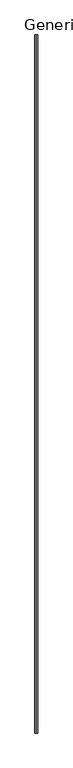
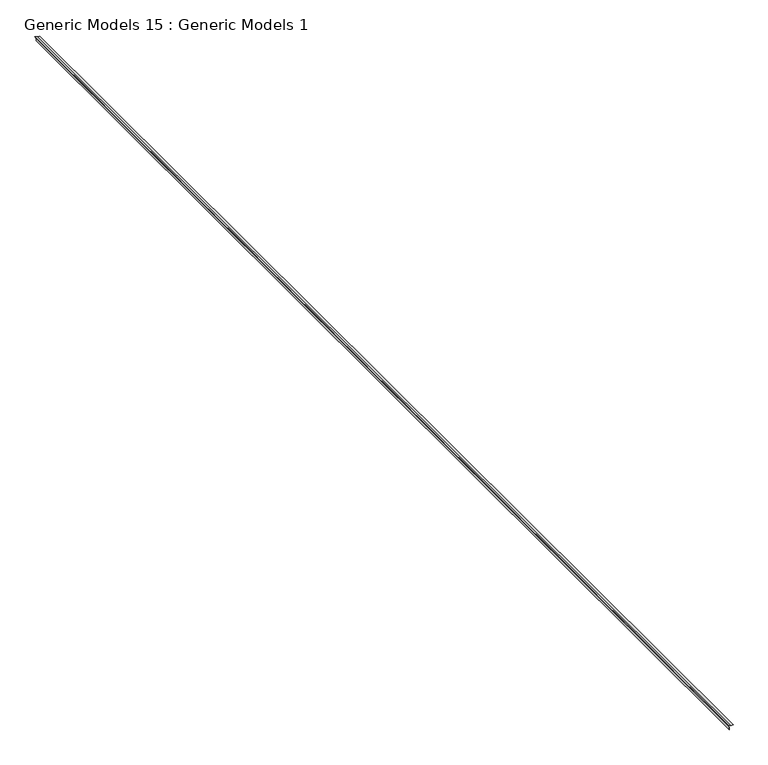
"""IFC4 building model written with IfcOpenShell, lengths in millimetres: proxy geometry, Generic Models 15 : Generic Models 1."""

from ifc_helpers import new_model, si_unit, point, frame, frame_2d, origin, place, context, project, spatial, polyline, circle_curve, trimmed, segment, composite_curve, outline, extrude, source, transform, mapped, element, save


def generic_models_15_generic_models_1_eb5eed79(model_context):
    return source(origin(), model_context, "Body", "SweptSolid", [
        extrude(outline(composite_curve([segment(trimmed(circle_curve(frame_2d((127127.2167873, 8355.8457008)), 1.4342127), [point((127128.4926156, 8356.5008558))], [point((127126.5616323, 8354.5698725))], False, "CARTESIAN"), True, "CONTINUOUS"), segment(polyline([(127126.5616323, 8354.5698725), (127088.5361176, 8374.0964881), (127050.4361176, 8374.0964881), (127050.4361176, 8375.3664881), (127088.8431414, 8375.3664881), (127127.5962396, 8355.4662484), (127107.696, 8394.2193467), (127107.696, 8432.6263704), (127108.966, 8432.6263704), (127108.966, 8394.5263704), (127128.4926156, 8356.5008558)]), True, "CONTINUOUS")], self_intersect=False)), frame((0.0, -7068.1230338, 0.0), z_axis=(0.0, 1.0, 0.0), x_axis=(0.0, 0.0, 1.0)), (0.0, 0.0, 1.0), 19050.0),
    ])


if __name__ == "__main__":
    model = new_model("IFC4")
    model_context = context("Model", 3, world=origin())
    ifc_project = project(units=[si_unit("LENGTHUNIT", "METRE", prefix="MILLI")], contexts=[model_context])
    site = spatial("IfcSite", under=ifc_project)
    building = spatial("IfcBuilding", under=site)
    placement = place(None, origin())
    generic_models_15_generic_models_1_shape = generic_models_15_generic_models_1_eb5eed79(model_context)
    element("IfcBuildingElementProxy", 1, Name="Generic Models 15 : Generic Models 1", ObjectType="Generic Models 15 : Generic Models 1", at=placement, inside=building, context=model_context, shape_type="MappedRepresentation", body=[
        mapped(generic_models_15_generic_models_1_shape, transform((0.0, 0.0, 0.0), x_axis=(1.0, 0.0, 0.0), y_axis=(0.0, 1.0, 0.0), z_axis=(0.0, 0.0, 1.0))),
    ])
    save(model, "model.ifc")

# Revit data of these elements
# Element 1 (IfcBuildingElementProxy, "Generic Models 15 : Generic Models 1")
#   Materials on its faces: "_CONTINUOUS 16 GA. COPPER CORNER BEAD"
# Materials
#   "_CONTINUOUS 16 GA. COPPER CORNER BEAD": class "Generic", colour RGB 253 192 103, transparency 0, Cost = 0
